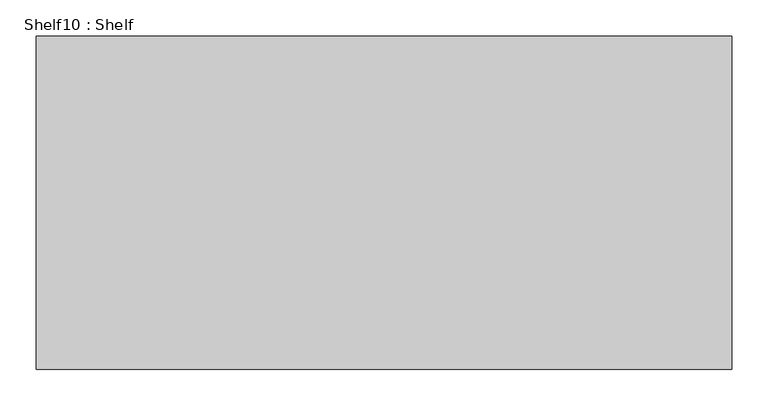
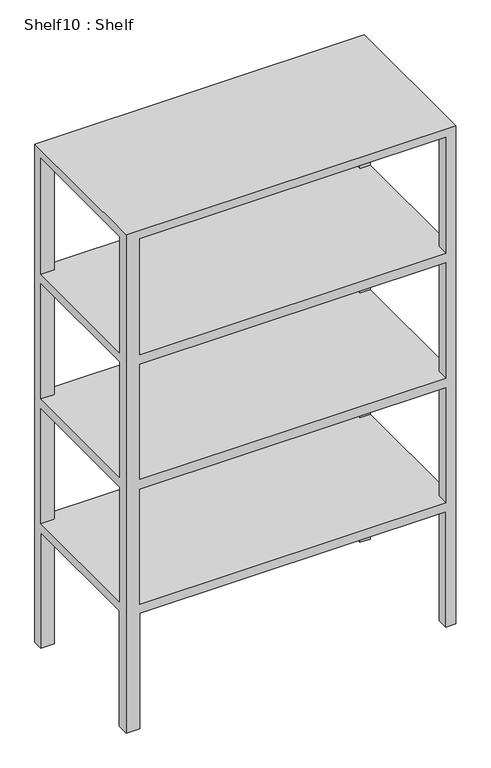
"""IFC4 building model written with IfcOpenShell, lengths in millimetres: furniture geometry, Shelf10 : Shelf."""

from ifc_helpers import new_model, si_unit, origin, place, context, project, spatial, faceted_brep, source, transform, mapped, element, save


def shelf10_shelf_d6147bd8(model_context):
    return source(origin(), model_context, "Body", "Brep", [
        faceted_brep([(14056.7001442, 10948.6615366, 1524.0), (14056.7001442, 11405.8615366, 1524.0), (13103.4798744, 11405.8615366, 1524.0), (13103.4798744, 10948.6615366, 1524.0), (14056.7001442, 10948.6615366, 0.0), (14028.3529362, 10948.6615366, 0.0), (14028.3529362, 10981.2181796, 0.0), (14056.7001442, 10981.2181796, 0.0), (14027.0281946, 11405.8615366, 0.0), (14056.7001442, 11405.8615366, 0.0), (14056.7001442, 11376.9377422, 0.0), (14027.0281946, 11376.9377422, 0.0), (13142.3001442, 10948.6615366, 0.0), (13103.4798744, 10948.6615366, 0.0), (13103.4798744, 10982.4555128, 0.0), (13142.3001442, 10982.4555128, 0.0), (13103.4798744, 11376.9377422, 0.0), (13103.4798744, 11405.8615366, 0.0), (13142.3001442, 11405.8615366, 0.0), (13142.3001442, 11376.9377422, 0.0), (13142.3001442, 10948.6615366, 353.3332002), (14028.3529362, 10948.6615366, 353.3332002), (13142.3001442, 10948.6615366, 1497.6781444), (14028.3529362, 10948.6615366, 1497.6781444), (14028.3529362, 10948.6615366, 1143.0), (13142.3001442, 10948.6615366, 1143.0), (13142.3001442, 10948.6615366, 1114.8196695), (14028.3529362, 10948.6615366, 1114.8196695), (14028.3529362, 10948.6615366, 762.0), (13142.3001442, 10948.6615366, 762.0), (13142.3001442, 10948.6615366, 731.9611947), (14028.3529362, 10948.6615366, 731.9611947), (14028.3529362, 10948.6615366, 381.0), (13142.3001442, 10948.6615366, 381.0), (13103.4798744, 11376.9377422, 353.3332002), (13103.4798744, 10982.4555128, 353.3332002), (13103.4798744, 11376.9377422, 1497.6781444), (13103.4798744, 10982.4555128, 1497.6781444), (13103.4798744, 10982.4555128, 1143.0), (13103.4798744, 11376.9377422, 1143.0), (13103.4798744, 11376.9377422, 1114.8196695), (13103.4798744, 10982.4555128, 1114.8196695), (13103.4798744, 10982.4555128, 762.0), (13103.4798744, 11376.9377422, 762.0), (13103.4798744, 11376.9377422, 731.9611947), (13103.4798744, 10982.4555128, 731.9611947), (13103.4798744, 10982.4555128, 381.0), (13103.4798744, 11376.9377422, 381.0), (14027.0281946, 11405.8615366, 353.3332002), (13142.3001442, 11405.8615366, 353.3332002), (14027.0281946, 11405.8615366, 1497.6781444), (13142.3001442, 11405.8615366, 1497.6781444), (13142.3001442, 11405.8615366, 1143.0), (14027.0281946, 11405.8615366, 1143.0), (14027.0281946, 11405.8615366, 1114.8196695), (13142.3001442, 11405.8615366, 1114.8196695), (13142.3001442, 11405.8615366, 762.0), (14027.0281946, 11405.8615366, 762.0), (14027.0281946, 11405.8615366, 731.9611947), (13142.3001442, 11405.8615366, 731.9611947), (13142.3001442, 11405.8615366, 381.0), (14027.0281946, 11405.8615366, 381.0), (14056.7001442, 10981.2181796, 353.3332002), (14056.7001442, 11376.9377422, 353.3332002), (14056.7001442, 10981.2181796, 1497.6781444), (14056.7001442, 11376.9377422, 1497.6781444), (14056.7001442, 11376.9377422, 1143.0), (14056.7001442, 10981.2181796, 1143.0), (14056.7001442, 10981.2181796, 1114.8196695), (14056.7001442, 11376.9377422, 1114.8196695), (14056.7001442, 11376.9377422, 762.0), (14056.7001442, 10981.2181796, 762.0), (14056.7001442, 10981.2181796, 731.9611947), (14056.7001442, 11376.9377422, 731.9611947), (14056.7001442, 11376.9377422, 381.0), (14056.7001442, 10981.2181796, 381.0), (13142.3001442, 11376.9377422, 1497.6781444), (14027.0281946, 11376.9377422, 1497.6781444), (14028.3529362, 10981.2181796, 1497.6781444), (13142.3001442, 10982.4555128, 1497.6781444), (13142.3001442, 11376.9377422, 1143.0), (13142.3001442, 10982.4555128, 1143.0), (14028.3529362, 10981.2181796, 1143.0), (14027.0281946, 11376.9377422, 1143.0), (13142.3001442, 11376.9377422, 1114.8196695), (14027.0281946, 11376.9377422, 1114.8196695), (14028.3529362, 10981.2181796, 1114.8196695), (13142.3001442, 10982.4555128, 1114.8196695), (13142.3001442, 11376.9377422, 762.0), (13142.3001442, 10982.4555128, 762.0), (14028.3529362, 10981.2181796, 762.0), (14027.0281946, 11376.9377422, 762.0), (13142.3001442, 11376.9377422, 731.9611947), (14027.0281946, 11376.9377422, 731.9611947), (14028.3529362, 10981.2181796, 731.9611947), (13142.3001442, 10982.4555128, 731.9611947), (13142.3001442, 11376.9377422, 381.0), (13142.3001442, 10982.4555128, 381.0), (14028.3529362, 10981.2181796, 381.0), (14027.0281946, 11376.9377422, 381.0), (13142.3001442, 11376.9377422, 353.3332002), (14027.0281946, 11376.9377422, 353.3332002), (14028.3529362, 10981.2181796, 353.3332002), (13142.3001442, 10982.4555128, 353.3332002)], [[[0, 1, 2, 3]], [[4, 5, 6, 7]], [[8, 9, 10, 11]], [[12, 13, 14, 15]], [[16, 17, 18, 19]], [[0, 3, 13, 12, 20, 21, 5, 4], [22, 23, 24, 25], [26, 27, 28, 29], [30, 31, 32, 33]], [[3, 2, 17, 16, 34, 35, 14, 13], [36, 37, 38, 39], [40, 41, 42, 43], [44, 45, 46, 47]], [[2, 1, 9, 8, 48, 49, 18, 17], [50, 51, 52, 53], [54, 55, 56, 57], [58, 59, 60, 61]], [[1, 0, 4, 7, 62, 63, 10, 9], [64, 65, 66, 67], [68, 69, 70, 71], [72, 73, 74, 75]], [[76, 51, 50, 77, 65, 64, 78, 23, 22, 79, 37, 36]], [[80, 39, 38, 81, 25, 24, 82, 67, 66, 83, 53, 52]], [[51, 76, 80, 52]], [[77, 50, 53, 83]], [[65, 77, 83, 66]], [[78, 64, 67, 82]], [[23, 78, 82, 24]], [[79, 22, 25, 81]], [[37, 79, 81, 38]], [[76, 36, 39, 80]], [[84, 55, 54, 85, 69, 68, 86, 27, 26, 87, 41, 40]], [[88, 43, 42, 89, 29, 28, 90, 71, 70, 91, 57, 56]], [[55, 84, 88, 56]], [[85, 54, 57, 91]], [[69, 85, 91, 70]], [[86, 68, 71, 90]], [[27, 86, 90, 28]], [[87, 26, 29, 89]], [[41, 87, 89, 42]], [[84, 40, 43, 88]], [[92, 59, 58, 93, 73, 72, 94, 31, 30, 95, 45, 44]], [[96, 47, 46, 97, 33, 32, 98, 75, 74, 99, 61, 60]], [[59, 92, 96, 60]], [[93, 58, 61, 99]], [[73, 93, 99, 74]], [[94, 72, 75, 98]], [[31, 94, 98, 32]], [[95, 30, 33, 97]], [[45, 95, 97, 46]], [[92, 44, 47, 96]], [[100, 49, 48, 101, 63, 62, 102, 21, 20, 103, 35, 34]], [[49, 100, 19, 18]], [[101, 48, 8, 11]], [[63, 101, 11, 10]], [[102, 62, 7, 6]], [[21, 102, 6, 5]], [[103, 20, 12, 15]], [[35, 103, 15, 14]], [[100, 34, 16, 19]]]),
    ])


if __name__ == "__main__":
    model = new_model("IFC4")
    model_context = context("Model", 3, world=origin())
    ifc_project = project(units=[si_unit("LENGTHUNIT", "METRE", prefix="MILLI")], contexts=[model_context])
    site = spatial("IfcSite", under=ifc_project)
    building = spatial("IfcBuilding", under=site)
    placement = place(None, origin())
    shelf10_shelf_shape = shelf10_shelf_d6147bd8(model_context)
    element("IfcFurniture", 1, ObjectType="Shelf10 : Shelf", at=placement, inside=building, context=model_context, shape_type="MappedRepresentation", body=[
        mapped(shelf10_shelf_shape, transform((0.0, 0.0, 0.0), x_axis=(1.0, 0.0, 0.0), y_axis=(0.0, 1.0, 0.0), z_axis=(0.0, 0.0, 1.0))),
    ])
    save(model, "model.ifc")
